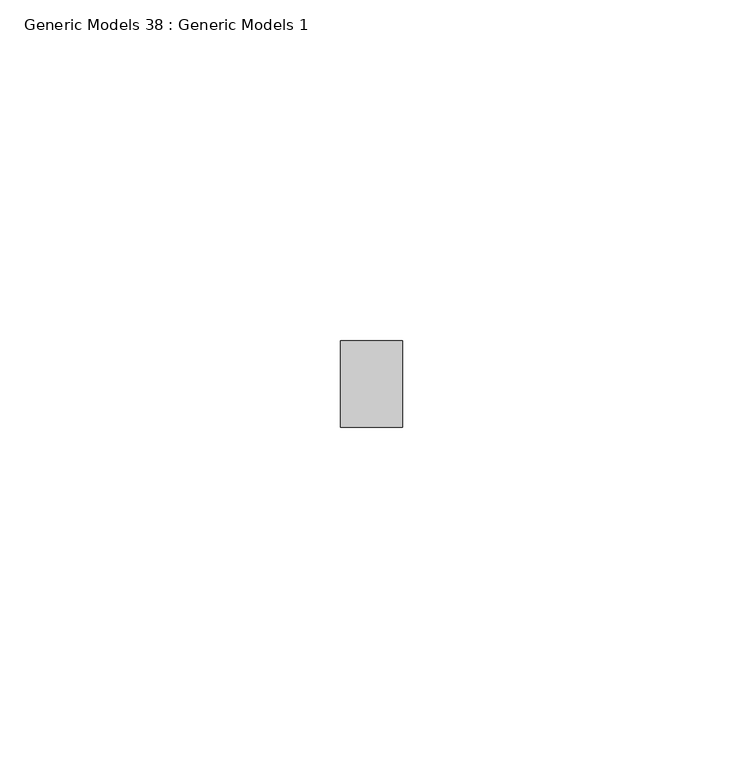
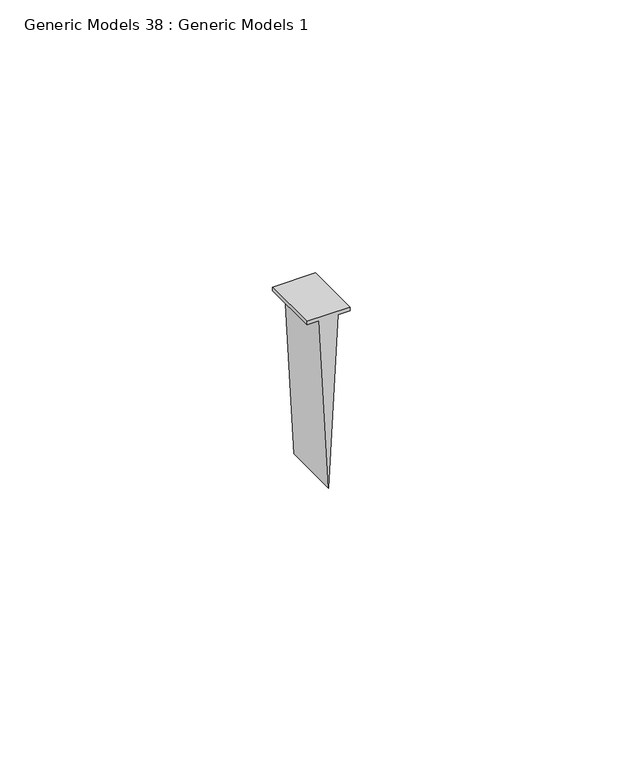
"""IFC4 building model written with IfcOpenShell, lengths in millimetres: proxy geometry, Generic Models 38 : Generic Models 1."""

from ifc_helpers import new_model, si_unit, frame, origin, place, context, project, spatial, polyline, outline, extrude, source, transform, mapped, element, save


def generic_models_38_generic_models_1_054f0e14(model_context):
    return source(origin(), model_context, "Body", "SweptSolid", [
        extrude(outline(polyline([(2443.027413, 49845.474547), (2442.233663, 49845.474547), (2442.233663, 49848.0244106), (2404.133663, 49850.021147), (2442.233663, 49852.0178834), (2442.233663, 49854.567747), (2443.027413, 49854.567747), (2443.027413, 49845.474547)])), frame((0.0, 565.15, 0.0), z_axis=(0.0, 1.0, 0.0), x_axis=(0.0, 0.0, 1.0)), (0.0, 0.0, 1.0), 12.7),
    ])


if __name__ == "__main__":
    model = new_model("IFC4")
    model_context = context("Model", 3, world=origin())
    ifc_project = project(units=[si_unit("LENGTHUNIT", "METRE", prefix="MILLI")], contexts=[model_context])
    site = spatial("IfcSite", under=ifc_project)
    building = spatial("IfcBuilding", under=site)
    placement = place(None, origin())
    generic_models_38_generic_models_1_shape = generic_models_38_generic_models_1_054f0e14(model_context)
    element("IfcBuildingElementProxy", 1, Name="Generic Models 38 : Generic Models 1", ObjectType="Generic Models 38 : Generic Models 1", at=placement, inside=building, context=model_context, shape_type="MappedRepresentation", body=[
        mapped(generic_models_38_generic_models_1_shape, transform((0.0, 0.0, 0.0), x_axis=(1.0, 0.0, 0.0), y_axis=(0.0, 1.0, 0.0), z_axis=(0.0, 0.0, 1.0))),
    ])
    save(model, "model.ifc")

# Revit data of these elements
# Element 1 (IfcBuildingElementProxy, "Generic Models 38 : Generic Models 1")
#   Materials on its faces: "ATTACH GYPSUM BOARD TO STUDS AND NOT TO TOP TRACK"
# Materials
#   "ATTACH GYPSUM BOARD TO STUDS AND NOT TO TOP TRACK": class "Generic", colour RGB 48 48 48, transparency 0, Cost = 0
